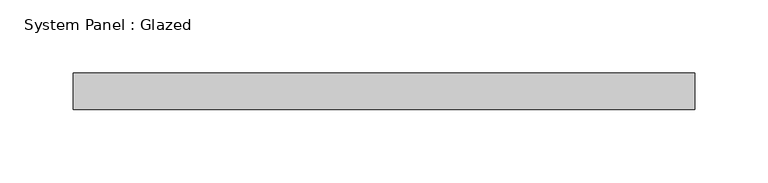
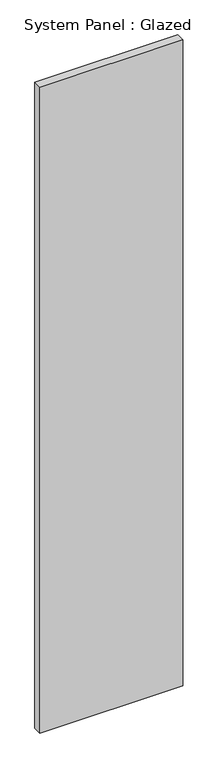
"""IFC4 building model written with IfcOpenShell, lengths in millimetres: plate geometry, System Panel : Glazed."""

import ifcopenshell
import ifcopenshell.guid

model = None  # the IFC model being written
_history = None  # IfcOwnerHistory: only IFC2X3 demands one
_inside = {}  # id of a spatial element -> (the spatial element, [elements in it])
_under = {}  # id of a project, library or spatial element -> (it, [spatial elements below it])
_declared = {}  # id of a project -> (the project, [libraries it declares])
_typed = {}  # id of a type object -> (the type object, [elements of that type])
_made_of = {}  # id of a material, layer set ... -> (it, [elements and type objects made of it])


def new_model(schema):
    """Start an empty IFC model of exactly this schema.

    Asked for "IFC4X3", IfcOpenShell would pick the latest addendum, in which some entities
    have other attributes; the version numbers below select the first issue.
    IFC2X3 requires an IfcOwnerHistory on every rooted entity: one is made here for all.
    """
    global model, _history
    if schema == "IFC4X3":
        model = ifcopenshell.file(schema_version=(4, 3, 0, 0))
    else:
        model = ifcopenshell.file(schema=schema)
    _inside.clear()
    _under.clear()
    _declared.clear()
    _typed.clear()
    _made_of.clear()
    _history = None
    if model.schema == "IFC2X3":
        org = make("IfcOrganization", Name="unknown")
        user = make(
            "IfcPersonAndOrganization",
            ThePerson=make("IfcPerson", FamilyName="unknown"),
            TheOrganization=org,
        )
        app = make(
            "IfcApplication",
            ApplicationDeveloper=org,
            Version="unknown",
            ApplicationFullName="unknown",
            ApplicationIdentifier="unknown",
        )
        _history = make(
            "IfcOwnerHistory",
            OwningUser=user,
            OwningApplication=app,
            ChangeAction="ADDED",
            CreationDate=0,
        )
    return model


def make(cls, **values):
    """One entity of the class cls with the attributes given. An attribute that is None is left unset."""
    return model.create_entity(
        cls, **{name: value for name, value in values.items() if value is not None}
    )


def rooted(cls, **values):
    """An entity with a GlobalId (a new one), such as an element, a storey or a relation."""
    return make(cls, GlobalId=ifcopenshell.guid.new(), OwnerHistory=_history, **values)


def si_unit(unit_type, name, prefix=None):
    """IfcSIUnit, for example si_unit("LENGTHUNIT", "METRE", prefix="MILLI")."""
    return make("IfcSIUnit", UnitType=unit_type, Prefix=prefix, Name=name)


def assignment(units):
    """IfcUnitAssignment: the units of a project."""
    return None if units is None else make("IfcUnitAssignment", Units=units)


def point(xyz):
    """IfcCartesianPoint."""
    return None if xyz is None else make("IfcCartesianPoint", Coordinates=xyz)


def direction(xyz):
    """IfcDirection."""
    return None if xyz is None else make("IfcDirection", DirectionRatios=xyz)


def frame(location, z_axis=None, x_axis=None):
    """IfcAxis2Placement3D, a coordinate frame: its origin and axes. An axis left out is left unset."""
    return make(
        "IfcAxis2Placement3D",
        Location=point(location),
        Axis=direction(z_axis),
        RefDirection=direction(x_axis),
    )


def origin():
    """The frame at (0, 0, 0) with its axes left unset."""
    return frame((0.0, 0.0, 0.0))


def origin_with_axes():
    """The frame at (0, 0, 0) with the z axis (0, 0, 1) and the x axis (1, 0, 0) written out."""
    return frame((0.0, 0.0, 0.0), z_axis=(0.0, 0.0, 1.0), x_axis=(1.0, 0.0, 0.0))


def place(relative_to, where):
    """IfcLocalPlacement: puts the frame where relative to a parent placement (None: the world)."""
    return make(
        "IfcLocalPlacement", PlacementRelTo=relative_to, RelativePlacement=where
    )


def context(
    kind, dimensions, precision=None, world=None, true_north=None, identifier=None
):
    """IfcGeometricRepresentationContext, for example the 3D "Model" context."""
    return make(
        "IfcGeometricRepresentationContext",
        ContextIdentifier=identifier,
        ContextType=kind,
        CoordinateSpaceDimension=dimensions,
        Precision=precision,
        WorldCoordinateSystem=world,
        TrueNorth=true_north,
    )


def project(units=None, contexts=None):
    """IfcProject with its units and contexts."""
    return rooted(
        "IfcProject",
        Name="project",
        RepresentationContexts=contexts,
        UnitsInContext=assignment(units),
    )


def spatial(cls, under=None, at=None, **own):
    """A site, building, storey or space (cls), placed at a placement, below another one or the project."""
    s = rooted(cls, ObjectPlacement=at, **own)
    if under is not None:
        _under.setdefault(under.id(), (under, []))[1].append(s)
    return s


def polyline(points):
    """IfcPolyline through the points."""
    return make("IfcPolyline", Points=[point(p) for p in points])


def outline(outer, holes=None, kind="AREA"):
    """IfcArbitraryClosedProfileDef: a profile drawn as a closed curve; with holes, ...WithVoids."""
    if holes is None:
        return make("IfcArbitraryClosedProfileDef", ProfileType=kind, OuterCurve=outer)
    return make(
        "IfcArbitraryProfileDefWithVoids",
        ProfileType=kind,
        OuterCurve=outer,
        InnerCurves=holes,
    )


def extrude(swept, where, along, depth):
    """IfcExtrudedAreaSolid: the profile swept, set in the frame where, extruded along a direction by depth."""
    return make(
        "IfcExtrudedAreaSolid",
        SweptArea=swept,
        Position=where,
        ExtrudedDirection=direction(along),
        Depth=depth,
    )


def shape(context_of_items, identifier, shape_type, items):
    """IfcShapeRepresentation: the items that make up one representation, for example the "Body"."""
    return make(
        "IfcShapeRepresentation",
        ContextOfItems=context_of_items,
        RepresentationIdentifier=identifier,
        RepresentationType=shape_type,
        Items=items,
    )


def source(mapping_origin, context_of_items, identifier, shape_type, items):
    """IfcRepresentationMap: a shape defined once, which mapped items show again and again."""
    return make(
        "IfcRepresentationMap",
        MappingOrigin=mapping_origin,
        MappedRepresentation=shape(context_of_items, identifier, shape_type, items),
    )


def transform(
    local_origin,
    x_axis=None,
    y_axis=None,
    z_axis=None,
    scale=None,
    scale2=None,
    scale3=None,
    uniform=True,
):
    """IfcCartesianTransformationOperator3D, or its non-uniform kind. x_axis, y_axis, z_axis: its Axis1, 2, 3."""
    if uniform:
        return make(
            "IfcCartesianTransformationOperator3D",
            Axis1=direction(x_axis),
            Axis2=direction(y_axis),
            LocalOrigin=point(local_origin),
            Scale=scale,
            Axis3=direction(z_axis),
        )
    return make(
        "IfcCartesianTransformationOperator3DnonUniform",
        Axis1=direction(x_axis),
        Axis2=direction(y_axis),
        LocalOrigin=point(local_origin),
        Scale=scale,
        Axis3=direction(z_axis),
        Scale2=scale2,
        Scale3=scale3,
    )


def mapped(mapping_source, mapping_target):
    """IfcMappedItem: shows the shape of a source again, moved by a transform."""
    return make(
        "IfcMappedItem", MappingSource=mapping_source, MappingTarget=mapping_target
    )


def made_of(thing, what):
    """Note that an element or type object is made of a material, layer set ...; save() writes the relation."""
    if what is not None:
        _made_of.setdefault(what.id(), (what, []))[1].append(thing)
    return thing


def element(
    cls,
    number,
    at=None,
    inside=None,
    cuts=None,
    type_object=None,
    material=None,
    context=None,
    identifier="Body",
    shape_type=None,
    held_by="IfcProductDefinitionShape",
    body=None,
    shapes=None,
    **own,
):
    """One element of the class cls, such as IfcWall. Its Tag is "e" and its number.

    at: its placement. inside: the storey or other place that contains it. cuts: it is an
    opening in that element (IfcRelVoidsElement). A single representation is given by context,
    identifier, shape_type and body (its items); several are given by shapes. held_by: the class
    of the entity that holds the representations. save() writes the other relations.
    """
    e = rooted(cls, Tag="e%d" % number, ObjectPlacement=at, **own)
    if body is not None:
        shapes = [shape(context, identifier, shape_type, body)]
    if shapes is not None:
        e.Representation = make(held_by, Representations=shapes)
    if inside is not None:
        _inside.setdefault(inside.id(), (inside, []))[1].append(e)
    if cuts is not None:
        rooted(
            "IfcRelVoidsElement", RelatingBuildingElement=cuts, RelatedOpeningElement=e
        )
    if type_object is not None:
        _typed.setdefault(type_object.id(), (type_object, []))[1].append(e)
    return made_of(e, material)


def aggregate(whole, parts):
    """IfcRelAggregates: a whole, such as a stair, and the parts it consists of."""
    return rooted("IfcRelAggregates", RelatingObject=whole, RelatedObjects=parts)


def save(model, path):
    """Write the relations noted so far, then the file.

    IfcRelAggregates (storeys below a building ...), IfcRelContainedInSpatialStructure (elements
    in a storey), IfcRelDefinesByType, IfcRelAssociatesMaterial and IfcRelDeclares: one each for
    every whole, place, type object, material and project.
    """
    for whole, parts in _under.values():
        aggregate(whole, parts)
    for where, things in _inside.values():
        rooted(
            "IfcRelContainedInSpatialStructure",
            RelatedElements=things,
            RelatingStructure=where,
        )
    for kind, things in _typed.values():
        rooted("IfcRelDefinesByType", RelatedObjects=things, RelatingType=kind)
    for what, things in _made_of.values():
        rooted("IfcRelAssociatesMaterial", RelatedObjects=things, RelatingMaterial=what)
    for by, libraries in _declared.values():
        rooted("IfcRelDeclares", RelatingContext=by, RelatedDefinitions=libraries)
    model.write(path)


def system_panel_glazed_248dfa94(model_context):
    return source(origin(), model_context, "Body", "SweptSolid", [
        extrude(outline(polyline([(212.5000001, 24.5), (-212.5000001, 24.5), (-212.5000001, 49.5), (212.5000001, 49.5), (212.5000001, 24.5)])), origin_with_axes(), (0.0, 0.0, 1.0), 2030.4462072),
    ])


if __name__ == "__main__":
    model = new_model("IFC4")
    model_context = context("Model", 3, world=origin())
    ifc_project = project(units=[si_unit("LENGTHUNIT", "METRE", prefix="MILLI")], contexts=[model_context])
    site = spatial("IfcSite", under=ifc_project)
    building = spatial("IfcBuilding", under=site)
    placement = place(None, origin())
    system_panel_glazed_shape = system_panel_glazed_248dfa94(model_context)
    element("IfcPlate", 1, ObjectType="System Panel : Glazed", at=placement, inside=building, context=model_context, shape_type="MappedRepresentation", body=[
        mapped(system_panel_glazed_shape, transform((0.0, 0.0, 0.0), x_axis=(1.0, 0.0, 0.0), y_axis=(0.0, 1.0, 0.0), z_axis=(0.0, 0.0, 1.0))),
    ])
    save(model, "model.ifc")

# Revit data of these elements
# Type "System Panel : Glazed"
#   Construction Type Id = "GSP4R"
#   Analytic Construction = "1/8 in Pilkington single glazing"
#   Visual Light Transmittance = 0.9
#   Solar Heat Gain Coefficient = 0.86
#   Heat Transfer Coefficient (U) = 6.7069 W/(m²·K)
#   Define Thermal Properties by = 1
# Element 1 (IfcPlate, "System Panel : Glazed")
#   Materials on its faces: "Glass"
# Materials
#   "Glass": class "Glass", colour RGB 0 128 192, transparency 0.9, Description = "Soda Lime Glass", Cost = 0
